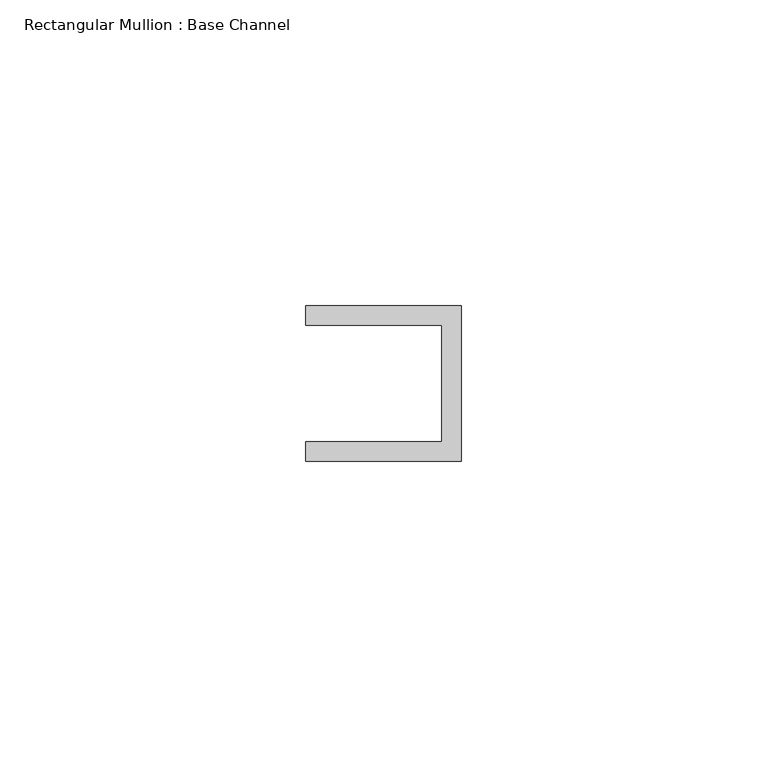
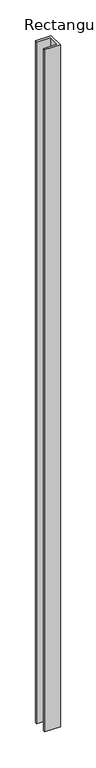
"""IFC4 building model written with IfcOpenShell, lengths in millimetres: member geometry, Rectangular Mullion : Base Channel."""

from ifc_helpers import new_model, si_unit, frame, origin, place, context, project, spatial, polyline, outline, extrude, source, transform, mapped, element, save


def rectangular_mullion_base_channel_0119d169(model_context):
    return source(origin(), model_context, "Body", "SweptSolid", [
        extrude(outline(polyline([(0.0, -12.7), (-25.4, -12.7), (-25.4, -9.525), (-3.175, -9.525), (-3.175, 9.525), (-25.4, 9.525), (-25.4, 12.7), (0.0, 12.7), (0.0, -12.7)])), frame((0.0, 0.0, -1165.225), z_axis=(0.0, 0.0, 1.0), x_axis=(1.0, 0.0, 0.0)), (0.0, 0.0, 1.0), 1165.225),
    ])


if __name__ == "__main__":
    model = new_model("IFC4")
    model_context = context("Model", 3, world=origin())
    ifc_project = project(units=[si_unit("LENGTHUNIT", "METRE", prefix="MILLI")], contexts=[model_context])
    site = spatial("IfcSite", under=ifc_project)
    building = spatial("IfcBuilding", under=site)
    placement = place(None, origin())
    rectangular_mullion_base_channel_shape = rectangular_mullion_base_channel_0119d169(model_context)
    element("IfcMember", 1, ObjectType="Rectangular Mullion : Base Channel", at=placement, inside=building, context=model_context, shape_type="MappedRepresentation", body=[
        mapped(rectangular_mullion_base_channel_shape, transform((0.0, 0.0, 0.0), x_axis=(1.0, 0.0, 0.0), y_axis=(0.0, 1.0, 0.0), z_axis=(0.0, 0.0, 1.0))),
    ])
    save(model, "model.ifc")

# Revit data of these elements
# Project information
#   Project Issue Date = "Issue Date"
#   Project Status = "Project Status"
#   Client Name = "Owner"
#   Project Address = "Enter address here"
#   Project Name = "1 S Pinkney St    Suite 340 Conference Room"
#   Project Number = "Project Number"
# Type "Rectangular Mullion : Base Channel"
#   built-in parameter 1007322 = 0.0833333 (stored number, unit not read)
#   built-in parameter 1007321 = 0.0416667 (stored number, unit not read)
#   built-in parameter 1007320 = -0.03125 (stored number, unit not read)
# Element 1 (IfcMember, "Rectangular Mullion : Base Channel")
#   Materials on its faces: "ALUM"
# Materials
#   "ALUM": class "Generic", colour RGB 157 157 157, transparency 0, Cost = 0
